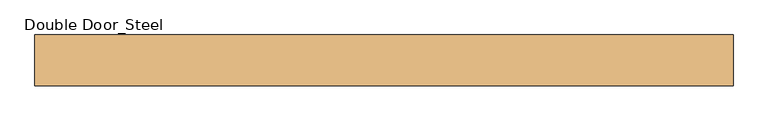
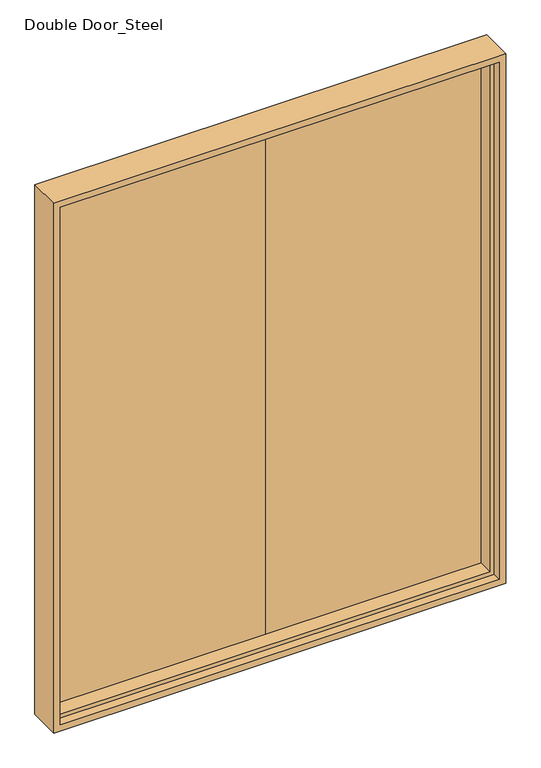
"""IFC4 building model written with IfcOpenShell, lengths in millimetres: door geometry, Double Door_Steel : H_DR_AR B12_Door_Double_W2100xH2580_FR 1.0H_FSD-5."""

from ifc_helpers import new_model, si_unit, frame, origin, place, context, project, spatial, polyline, outline, extrude, faceted_brep, source, transform, mapped, element, save


def double_door_steel_b4304629(model_context):
    return source(origin(), model_context, "Body", "SolidModel", [
        faceted_brep([(-1035.0, -75.0, 2565.0), (-1035.0, 75.0, 2565.0), (-1035.0, 75.0, 0.0), (-1035.0, -75.0, 0.0), (1035.0, 75.0, 0.0), (1035.0, 75.0, 2565.0), (1005.0, 75.0, 2535.0), (-1005.0, 75.0, 2535.0), (-1005.0, 75.0, 30.0), (1005.0, 75.0, 30.0), (1035.0, -75.0, 0.0), (1035.0, -75.0, 2565.0), (1005.0, -75.0, 30.0), (-1005.0, -75.0, 30.0), (-1005.0, -75.0, 2535.0), (1005.0, -75.0, 2535.0), (-1005.0, -35.0, 2535.0), (-1005.0, -35.0, 30.0), (1005.0, -35.0, 30.0), (1005.0, -35.0, 2535.0), (985.0, -35.0, 2515.0), (985.0, -35.0, 50.0), (-985.0, -35.0, 50.0), (-985.0, -35.0, 2515.0), (-985.0, 35.0, 2515.0), (-985.0, 35.0, 50.0), (985.0, 35.0, 50.0), (1005.0, 35.0, 30.0), (-1005.0, 35.0, 30.0), (-1005.0, 35.0, 2535.0), (1005.0, 35.0, 2535.0), (985.0, 35.0, 2515.0)], [[[0, 1, 2, 3]], [[4, 2, 1, 5], [6, 7, 8, 9]], [[3, 2, 4, 10]], [[11, 0, 3, 10], [12, 13, 14, 15]], [[16, 14, 13, 17]], [[17, 13, 12, 18]], [[16, 17, 18, 19], [20, 21, 22, 23]], [[24, 23, 22, 25]], [[25, 22, 21, 26]], [[27, 28, 29, 30], [31, 24, 25, 26]], [[7, 29, 28, 8]], [[8, 28, 27, 9]], [[10, 4, 5, 11]], [[9, 27, 30, 6]], [[18, 12, 15, 19]], [[26, 21, 20, 31]], [[11, 5, 1, 0]], [[19, 15, 14, 16]], [[31, 20, 23, 24]], [[6, 30, 29, 7]]]),
        extrude(outline(polyline([(1005.0, 35.0), (0.0, 35.0), (0.0, 75.0), (1005.0, 75.0), (1005.0, 35.0)])), frame((0.0, 0.0, 30.0), z_axis=(0.0, 0.0, 1.0), x_axis=(1.0, 0.0, 0.0)), (0.0, 0.0, 1.0), 2505.0),
        extrude(outline(polyline([(0.0, 35.0), (-1005.0, 35.0), (-1005.0, 75.0), (0.0, 75.0), (0.0, 35.0)])), frame((0.0, 0.0, 30.0), z_axis=(0.0, 0.0, 1.0), x_axis=(1.0, 0.0, 0.0)), (0.0, 0.0, 1.0), 2505.0),
    ])


if __name__ == "__main__":
    model = new_model("IFC4")
    model_context = context("Model", 3, world=origin())
    ifc_project = project(units=[si_unit("LENGTHUNIT", "METRE", prefix="MILLI")], contexts=[model_context])
    site = spatial("IfcSite", under=ifc_project)
    building = spatial("IfcBuilding", under=site)
    placement = place(None, origin())
    double_door_steel_shape = double_door_steel_b4304629(model_context)
    element("IfcDoor", 1, ObjectType="Double Door_Steel : H_DR_AR B12_Door_Double_W2100xH2580_FR 1.0H_FSD-5", at=placement, inside=building, context=model_context, shape_type="MappedRepresentation", body=[
        mapped(double_door_steel_shape, transform((0.0, 0.0, 0.0), x_axis=(1.0, 0.0, 0.0), y_axis=(0.0, 1.0, 0.0), z_axis=(0.0, 0.0, 1.0))),
    ])
    save(model, "model.ifc")

# Revit data of these elements
# Type "Double Door_Steel : H_DR_AR B12_Door_Double_W2100xH2580_FR 1.0H_FSD-5"
#   Type Mark = "447"
#   프레임 = ""
#   철물 = ""
#   유리/마감 = ""
#   위치/개소 = ""
#   부호 = ""
#   문번호 = ""
#   문기호 = "FSD-4"
#   Analytic Construction = "<None>"
#   Door Width = 1005 mm
#   Height = 2580 mm
#   Width = 2100 mm
#   Define Thermal Properties by = 1
#   문 틀 = none
#   문 = none
#   Function = (empty or 0)
#   Assembly Code = ""
#   Wall Closure = (empty or 0)
